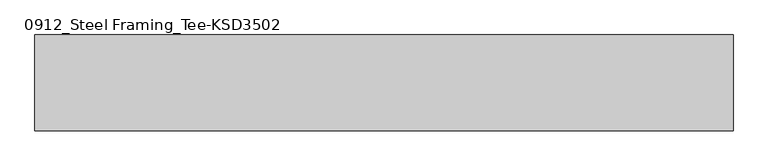
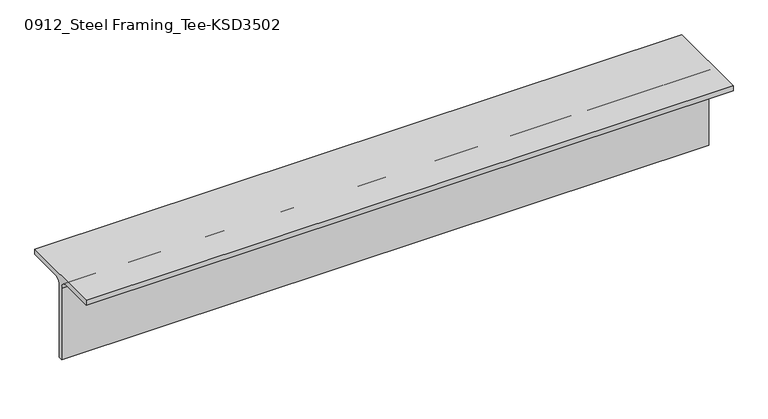
"""IFC4 building model written with IfcOpenShell, lengths in millimetres: member geometry, 0912_Steel Framing_Tee-KSD3502 : H_SB_ASB_CT-150x150x6.5x9."""

import ifcopenshell
import ifcopenshell.guid

model = None  # the IFC model being written
_history = None  # IfcOwnerHistory: only IFC2X3 demands one
_inside = {}  # id of a spatial element -> (the spatial element, [elements in it])
_under = {}  # id of a project, library or spatial element -> (it, [spatial elements below it])
_declared = {}  # id of a project -> (the project, [libraries it declares])
_typed = {}  # id of a type object -> (the type object, [elements of that type])
_made_of = {}  # id of a material, layer set ... -> (it, [elements and type objects made of it])


def new_model(schema):
    """Start an empty IFC model of exactly this schema.

    Asked for "IFC4X3", IfcOpenShell would pick the latest addendum, in which some entities
    have other attributes; the version numbers below select the first issue.
    IFC2X3 requires an IfcOwnerHistory on every rooted entity: one is made here for all.
    """
    global model, _history
    if schema == "IFC4X3":
        model = ifcopenshell.file(schema_version=(4, 3, 0, 0))
    else:
        model = ifcopenshell.file(schema=schema)
    _inside.clear()
    _under.clear()
    _declared.clear()
    _typed.clear()
    _made_of.clear()
    _history = None
    if model.schema == "IFC2X3":
        org = make("IfcOrganization", Name="unknown")
        user = make(
            "IfcPersonAndOrganization",
            ThePerson=make("IfcPerson", FamilyName="unknown"),
            TheOrganization=org,
        )
        app = make(
            "IfcApplication",
            ApplicationDeveloper=org,
            Version="unknown",
            ApplicationFullName="unknown",
            ApplicationIdentifier="unknown",
        )
        _history = make(
            "IfcOwnerHistory",
            OwningUser=user,
            OwningApplication=app,
            ChangeAction="ADDED",
            CreationDate=0,
        )
    return model


def make(cls, **values):
    """One entity of the class cls with the attributes given. An attribute that is None is left unset."""
    return model.create_entity(
        cls, **{name: value for name, value in values.items() if value is not None}
    )


def rooted(cls, **values):
    """An entity with a GlobalId (a new one), such as an element, a storey or a relation."""
    return make(cls, GlobalId=ifcopenshell.guid.new(), OwnerHistory=_history, **values)


def si_unit(unit_type, name, prefix=None):
    """IfcSIUnit, for example si_unit("LENGTHUNIT", "METRE", prefix="MILLI")."""
    return make("IfcSIUnit", UnitType=unit_type, Prefix=prefix, Name=name)


def assignment(units):
    """IfcUnitAssignment: the units of a project."""
    return None if units is None else make("IfcUnitAssignment", Units=units)


def point(xyz):
    """IfcCartesianPoint."""
    return None if xyz is None else make("IfcCartesianPoint", Coordinates=xyz)


def direction(xyz):
    """IfcDirection."""
    return None if xyz is None else make("IfcDirection", DirectionRatios=xyz)


def frame(location, z_axis=None, x_axis=None):
    """IfcAxis2Placement3D, a coordinate frame: its origin and axes. An axis left out is left unset."""
    return make(
        "IfcAxis2Placement3D",
        Location=point(location),
        Axis=direction(z_axis),
        RefDirection=direction(x_axis),
    )


def frame_2d(location, x_axis=None):
    """IfcAxis2Placement2D, a coordinate frame in the plane: its origin and x axis."""
    return make(
        "IfcAxis2Placement2D", Location=point(location), RefDirection=direction(x_axis)
    )


def origin():
    """The frame at (0, 0, 0) with its axes left unset."""
    return frame((0.0, 0.0, 0.0))


def place(relative_to, where):
    """IfcLocalPlacement: puts the frame where relative to a parent placement (None: the world)."""
    return make(
        "IfcLocalPlacement", PlacementRelTo=relative_to, RelativePlacement=where
    )


def context(
    kind, dimensions, precision=None, world=None, true_north=None, identifier=None
):
    """IfcGeometricRepresentationContext, for example the 3D "Model" context."""
    return make(
        "IfcGeometricRepresentationContext",
        ContextIdentifier=identifier,
        ContextType=kind,
        CoordinateSpaceDimension=dimensions,
        Precision=precision,
        WorldCoordinateSystem=world,
        TrueNorth=true_north,
    )


def project(units=None, contexts=None):
    """IfcProject with its units and contexts."""
    return rooted(
        "IfcProject",
        Name="project",
        RepresentationContexts=contexts,
        UnitsInContext=assignment(units),
    )


def spatial(cls, under=None, at=None, **own):
    """A site, building, storey or space (cls), placed at a placement, below another one or the project."""
    s = rooted(cls, ObjectPlacement=at, **own)
    if under is not None:
        _under.setdefault(under.id(), (under, []))[1].append(s)
    return s


def polyline(points):
    """IfcPolyline through the points."""
    return make("IfcPolyline", Points=[point(p) for p in points])


def circle_curve(where, radius):
    """IfcCircle in the frame where."""
    return make("IfcCircle", Position=where, Radius=radius)


def trimmed(basis, trim1, trim2, sense, master):
    """IfcTrimmedCurve: the piece of a basis curve between two trims."""
    return make(
        "IfcTrimmedCurve",
        BasisCurve=basis,
        Trim1=trim1,
        Trim2=trim2,
        SenseAgreement=sense,
        MasterRepresentation=master,
    )


def segment(curve, same_sense, transition):
    """IfcCompositeCurveSegment."""
    return make(
        "IfcCompositeCurveSegment",
        Transition=transition,
        SameSense=same_sense,
        ParentCurve=curve,
    )


def composite_curve(segments, self_intersect=None):
    """IfcCompositeCurve: segments joined end to end."""
    return make("IfcCompositeCurve", Segments=segments, SelfIntersect=self_intersect)


def outline(outer, holes=None, kind="AREA"):
    """IfcArbitraryClosedProfileDef: a profile drawn as a closed curve; with holes, ...WithVoids."""
    if holes is None:
        return make("IfcArbitraryClosedProfileDef", ProfileType=kind, OuterCurve=outer)
    return make(
        "IfcArbitraryProfileDefWithVoids",
        ProfileType=kind,
        OuterCurve=outer,
        InnerCurves=holes,
    )


def extrude(swept, where, along, depth):
    """IfcExtrudedAreaSolid: the profile swept, set in the frame where, extruded along a direction by depth."""
    return make(
        "IfcExtrudedAreaSolid",
        SweptArea=swept,
        Position=where,
        ExtrudedDirection=direction(along),
        Depth=depth,
    )


def shape(context_of_items, identifier, shape_type, items):
    """IfcShapeRepresentation: the items that make up one representation, for example the "Body"."""
    return make(
        "IfcShapeRepresentation",
        ContextOfItems=context_of_items,
        RepresentationIdentifier=identifier,
        RepresentationType=shape_type,
        Items=items,
    )


def source(mapping_origin, context_of_items, identifier, shape_type, items):
    """IfcRepresentationMap: a shape defined once, which mapped items show again and again."""
    return make(
        "IfcRepresentationMap",
        MappingOrigin=mapping_origin,
        MappedRepresentation=shape(context_of_items, identifier, shape_type, items),
    )


def transform(
    local_origin,
    x_axis=None,
    y_axis=None,
    z_axis=None,
    scale=None,
    scale2=None,
    scale3=None,
    uniform=True,
):
    """IfcCartesianTransformationOperator3D, or its non-uniform kind. x_axis, y_axis, z_axis: its Axis1, 2, 3."""
    if uniform:
        return make(
            "IfcCartesianTransformationOperator3D",
            Axis1=direction(x_axis),
            Axis2=direction(y_axis),
            LocalOrigin=point(local_origin),
            Scale=scale,
            Axis3=direction(z_axis),
        )
    return make(
        "IfcCartesianTransformationOperator3DnonUniform",
        Axis1=direction(x_axis),
        Axis2=direction(y_axis),
        LocalOrigin=point(local_origin),
        Scale=scale,
        Axis3=direction(z_axis),
        Scale2=scale2,
        Scale3=scale3,
    )


def mapped(mapping_source, mapping_target):
    """IfcMappedItem: shows the shape of a source again, moved by a transform."""
    return make(
        "IfcMappedItem", MappingSource=mapping_source, MappingTarget=mapping_target
    )


def made_of(thing, what):
    """Note that an element or type object is made of a material, layer set ...; save() writes the relation."""
    if what is not None:
        _made_of.setdefault(what.id(), (what, []))[1].append(thing)
    return thing


def element(
    cls,
    number,
    at=None,
    inside=None,
    cuts=None,
    type_object=None,
    material=None,
    context=None,
    identifier="Body",
    shape_type=None,
    held_by="IfcProductDefinitionShape",
    body=None,
    shapes=None,
    **own,
):
    """One element of the class cls, such as IfcWall. Its Tag is "e" and its number.

    at: its placement. inside: the storey or other place that contains it. cuts: it is an
    opening in that element (IfcRelVoidsElement). A single representation is given by context,
    identifier, shape_type and body (its items); several are given by shapes. held_by: the class
    of the entity that holds the representations. save() writes the other relations.
    """
    e = rooted(cls, Tag="e%d" % number, ObjectPlacement=at, **own)
    if body is not None:
        shapes = [shape(context, identifier, shape_type, body)]
    if shapes is not None:
        e.Representation = make(held_by, Representations=shapes)
    if inside is not None:
        _inside.setdefault(inside.id(), (inside, []))[1].append(e)
    if cuts is not None:
        rooted(
            "IfcRelVoidsElement", RelatingBuildingElement=cuts, RelatedOpeningElement=e
        )
    if type_object is not None:
        _typed.setdefault(type_object.id(), (type_object, []))[1].append(e)
    return made_of(e, material)


def aggregate(whole, parts):
    """IfcRelAggregates: a whole, such as a stair, and the parts it consists of."""
    return rooted("IfcRelAggregates", RelatingObject=whole, RelatedObjects=parts)


def save(model, path):
    """Write the relations noted so far, then the file.

    IfcRelAggregates (storeys below a building ...), IfcRelContainedInSpatialStructure (elements
    in a storey), IfcRelDefinesByType, IfcRelAssociatesMaterial and IfcRelDeclares: one each for
    every whole, place, type object, material and project.
    """
    for whole, parts in _under.values():
        aggregate(whole, parts)
    for where, things in _inside.values():
        rooted(
            "IfcRelContainedInSpatialStructure",
            RelatedElements=things,
            RelatingStructure=where,
        )
    for kind, things in _typed.values():
        rooted("IfcRelDefinesByType", RelatedObjects=things, RelatingType=kind)
    for what, things in _made_of.values():
        rooted("IfcRelAssociatesMaterial", RelatedObjects=things, RelatingMaterial=what)
    for by, libraries in _declared.values():
        rooted("IfcRelDeclares", RelatingContext=by, RelatedDefinitions=libraries)
    model.write(path)


def member_0912_steel_framing_tee_ksd3502_be89381c(model_context):
    return source(origin(), model_context, "Body", "SweptSolid", [
        extrude(outline(composite_curve([segment(polyline([(-75.0, 75.0), (75.0, 75.0), (75.0, 66.0), (16.25, 66.0)]), True, "CONTINUOUS"), segment(trimmed(circle_curve(frame_2d((16.25, 53.0)), 13.0), [point((16.25, 66.0))], [point((3.25, 53.0))], True, "CARTESIAN"), True, "CONTINUOUS"), segment(polyline([(3.25, 53.0), (3.25, -75.0), (-3.25, -75.0), (-3.25, 53.0)]), True, "CONTINUOUS"), segment(trimmed(circle_curve(frame_2d((-16.25, 53.0)), 13.0), [point((-3.25, 53.0))], [point((-16.25, 66.0))], True, "CARTESIAN"), True, "CONTINUOUS"), segment(polyline([(-16.25, 66.0), (-75.0, 66.0), (-75.0, 75.0)]), True, "CONTINUOUS")], self_intersect=False)), frame((-484.45, 0.0, 0.0), z_axis=(1.0, 0.0, 0.0), x_axis=(0.0, 1.0, 0.0)), (0.0, 0.0, 1.0), 1094.0),
    ])


if __name__ == "__main__":
    model = new_model("IFC4")
    model_context = context("Model", 3, world=origin())
    ifc_project = project(units=[si_unit("LENGTHUNIT", "METRE", prefix="MILLI")], contexts=[model_context])
    site = spatial("IfcSite", under=ifc_project)
    building = spatial("IfcBuilding", under=site)
    placement = place(None, origin())
    member_0912_steel_framing_tee_ksd3502_shape = member_0912_steel_framing_tee_ksd3502_be89381c(model_context)
    element("IfcMember", 1, ObjectType="0912_Steel Framing_Tee-KSD3502 : H_SB_ASB_CT-150x150x6.5x9", at=placement, inside=building, context=model_context, shape_type="MappedRepresentation", body=[
        mapped(member_0912_steel_framing_tee_ksd3502_shape, transform((0.0, 0.0, 0.0), x_axis=(1.0, 0.0, 0.0), y_axis=(0.0, 1.0, 0.0), z_axis=(0.0, 0.0, 1.0))),
    ])
    save(model, "model.ifc")

# Revit data of these elements
# Type "0912_Steel Framing_Tee-KSD3502 : H_SB_ASB_CT-150x150x6.5x9"
#   H_WM Code_1 = "S01AA003-00001 | Main Steel Structure Fabrication Work | Shelter/Building | Light Steel - Standard (30KG/M>Weight) | Material: (   )"
#   H_WM Code_2 = "S03AA029-00001 | Main Steel Structure Erection Work | Shelter/Building | Light Steel (30KG/M>Weight) | Material: (   )"
#   H_WM Code_3 = "S01AA010-00001 | Main Steel Structure Fabrication Work | Shelter/Building | Steel Painting/Coating | for Non-Fireproofed Steel Surface, Surface Preparation, Primer, Second & Final Coat | Material: (   )"
#   H_Q'ty Cal Type Tag = "SB-Q2"
#   Width = 15.0 cm
#   Web Thickness = 0.65 cm
#   Web Fillet = 1.3 cm
#   Section Area = 23.39 cm²
#   Perimeter = 0.60 m²/m
#   Nominal Weight = 18.40 kgf/m
#   Height = 15.0 cm
#   Flange Thickness = 0.9 cm
#   Centroid Vertical = 7.5 cm
#   Centroid Horizontal = 7.5 cm
#   Length [instance default] = 1.5000 m
#   Structural Material [instance default] = Steel, 45-345
#   Warping Constant = (empty or 0)
#   Torsional Moment of Inertia = 0
#   Section Name Key = ""
#   Plastic Modulus weak axis = 0
#   Plastic Modulus strong axis = 0
#   Moment of Inertia weak axis = 0
#   Moment of Inertia strong axis = 0
#   Elastic Modulus weak axis = 0
#   Elastic Modulus strong axis = 0
#   Bolt Spacing = 0
#   Assembly Code = ""
# Element 1 (IfcMember, "0912_Steel Framing_Tee-KSD3502 : H_SB_ASB_CT-150x150x6.5x9")
#   Structural Material = none
# Materials
#   "Steel, 45-345": class "Metal", colour RGB 189 187 185, transparency 0, Description = "Steel 345 MPa", Cost = 0
